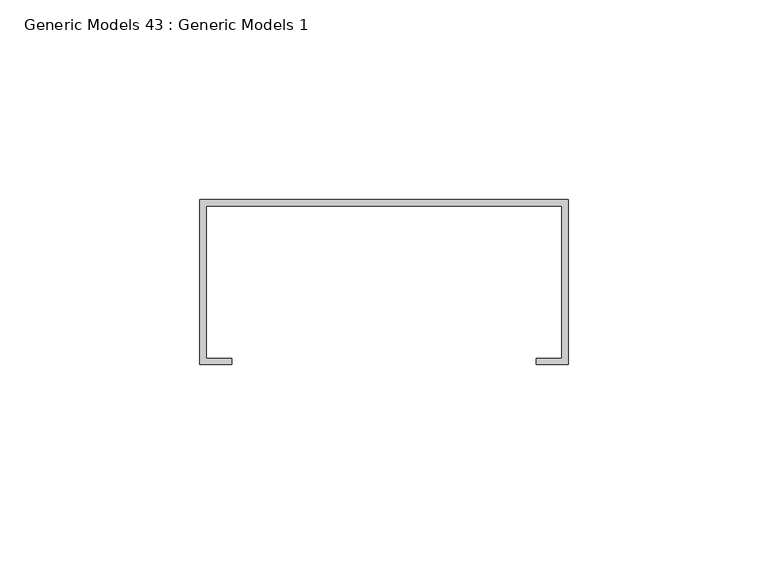
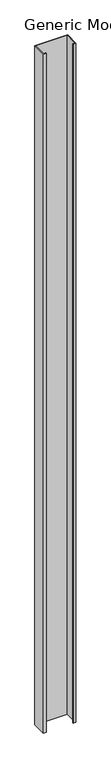
"""IFC4 building model written with IfcOpenShell, lengths in millimetres: proxy geometry, Generic Models 43 : Generic Models 1."""

import ifcopenshell
import ifcopenshell.guid

model = None  # the IFC model being written
_history = None  # IfcOwnerHistory: only IFC2X3 demands one
_inside = {}  # id of a spatial element -> (the spatial element, [elements in it])
_under = {}  # id of a project, library or spatial element -> (it, [spatial elements below it])
_declared = {}  # id of a project -> (the project, [libraries it declares])
_typed = {}  # id of a type object -> (the type object, [elements of that type])
_made_of = {}  # id of a material, layer set ... -> (it, [elements and type objects made of it])


def new_model(schema):
    """Start an empty IFC model of exactly this schema.

    Asked for "IFC4X3", IfcOpenShell would pick the latest addendum, in which some entities
    have other attributes; the version numbers below select the first issue.
    IFC2X3 requires an IfcOwnerHistory on every rooted entity: one is made here for all.
    """
    global model, _history
    if schema == "IFC4X3":
        model = ifcopenshell.file(schema_version=(4, 3, 0, 0))
    else:
        model = ifcopenshell.file(schema=schema)
    _inside.clear()
    _under.clear()
    _declared.clear()
    _typed.clear()
    _made_of.clear()
    _history = None
    if model.schema == "IFC2X3":
        org = make("IfcOrganization", Name="unknown")
        user = make(
            "IfcPersonAndOrganization",
            ThePerson=make("IfcPerson", FamilyName="unknown"),
            TheOrganization=org,
        )
        app = make(
            "IfcApplication",
            ApplicationDeveloper=org,
            Version="unknown",
            ApplicationFullName="unknown",
            ApplicationIdentifier="unknown",
        )
        _history = make(
            "IfcOwnerHistory",
            OwningUser=user,
            OwningApplication=app,
            ChangeAction="ADDED",
            CreationDate=0,
        )
    return model


def make(cls, **values):
    """One entity of the class cls with the attributes given. An attribute that is None is left unset."""
    return model.create_entity(
        cls, **{name: value for name, value in values.items() if value is not None}
    )


def rooted(cls, **values):
    """An entity with a GlobalId (a new one), such as an element, a storey or a relation."""
    return make(cls, GlobalId=ifcopenshell.guid.new(), OwnerHistory=_history, **values)


def si_unit(unit_type, name, prefix=None):
    """IfcSIUnit, for example si_unit("LENGTHUNIT", "METRE", prefix="MILLI")."""
    return make("IfcSIUnit", UnitType=unit_type, Prefix=prefix, Name=name)


def assignment(units):
    """IfcUnitAssignment: the units of a project."""
    return None if units is None else make("IfcUnitAssignment", Units=units)


def point(xyz):
    """IfcCartesianPoint."""
    return None if xyz is None else make("IfcCartesianPoint", Coordinates=xyz)


def direction(xyz):
    """IfcDirection."""
    return None if xyz is None else make("IfcDirection", DirectionRatios=xyz)


def frame(location, z_axis=None, x_axis=None):
    """IfcAxis2Placement3D, a coordinate frame: its origin and axes. An axis left out is left unset."""
    return make(
        "IfcAxis2Placement3D",
        Location=point(location),
        Axis=direction(z_axis),
        RefDirection=direction(x_axis),
    )


def origin():
    """The frame at (0, 0, 0) with its axes left unset."""
    return frame((0.0, 0.0, 0.0))


def place(relative_to, where):
    """IfcLocalPlacement: puts the frame where relative to a parent placement (None: the world)."""
    return make(
        "IfcLocalPlacement", PlacementRelTo=relative_to, RelativePlacement=where
    )


def context(
    kind, dimensions, precision=None, world=None, true_north=None, identifier=None
):
    """IfcGeometricRepresentationContext, for example the 3D "Model" context."""
    return make(
        "IfcGeometricRepresentationContext",
        ContextIdentifier=identifier,
        ContextType=kind,
        CoordinateSpaceDimension=dimensions,
        Precision=precision,
        WorldCoordinateSystem=world,
        TrueNorth=true_north,
    )


def project(units=None, contexts=None):
    """IfcProject with its units and contexts."""
    return rooted(
        "IfcProject",
        Name="project",
        RepresentationContexts=contexts,
        UnitsInContext=assignment(units),
    )


def spatial(cls, under=None, at=None, **own):
    """A site, building, storey or space (cls), placed at a placement, below another one or the project."""
    s = rooted(cls, ObjectPlacement=at, **own)
    if under is not None:
        _under.setdefault(under.id(), (under, []))[1].append(s)
    return s


def polyline(points):
    """IfcPolyline through the points."""
    return make("IfcPolyline", Points=[point(p) for p in points])


def outline(outer, holes=None, kind="AREA"):
    """IfcArbitraryClosedProfileDef: a profile drawn as a closed curve; with holes, ...WithVoids."""
    if holes is None:
        return make("IfcArbitraryClosedProfileDef", ProfileType=kind, OuterCurve=outer)
    return make(
        "IfcArbitraryProfileDefWithVoids",
        ProfileType=kind,
        OuterCurve=outer,
        InnerCurves=holes,
    )


def extrude(swept, where, along, depth):
    """IfcExtrudedAreaSolid: the profile swept, set in the frame where, extruded along a direction by depth."""
    return make(
        "IfcExtrudedAreaSolid",
        SweptArea=swept,
        Position=where,
        ExtrudedDirection=direction(along),
        Depth=depth,
    )


def shape(context_of_items, identifier, shape_type, items):
    """IfcShapeRepresentation: the items that make up one representation, for example the "Body"."""
    return make(
        "IfcShapeRepresentation",
        ContextOfItems=context_of_items,
        RepresentationIdentifier=identifier,
        RepresentationType=shape_type,
        Items=items,
    )


def source(mapping_origin, context_of_items, identifier, shape_type, items):
    """IfcRepresentationMap: a shape defined once, which mapped items show again and again."""
    return make(
        "IfcRepresentationMap",
        MappingOrigin=mapping_origin,
        MappedRepresentation=shape(context_of_items, identifier, shape_type, items),
    )


def transform(
    local_origin,
    x_axis=None,
    y_axis=None,
    z_axis=None,
    scale=None,
    scale2=None,
    scale3=None,
    uniform=True,
):
    """IfcCartesianTransformationOperator3D, or its non-uniform kind. x_axis, y_axis, z_axis: its Axis1, 2, 3."""
    if uniform:
        return make(
            "IfcCartesianTransformationOperator3D",
            Axis1=direction(x_axis),
            Axis2=direction(y_axis),
            LocalOrigin=point(local_origin),
            Scale=scale,
            Axis3=direction(z_axis),
        )
    return make(
        "IfcCartesianTransformationOperator3DnonUniform",
        Axis1=direction(x_axis),
        Axis2=direction(y_axis),
        LocalOrigin=point(local_origin),
        Scale=scale,
        Axis3=direction(z_axis),
        Scale2=scale2,
        Scale3=scale3,
    )


def mapped(mapping_source, mapping_target):
    """IfcMappedItem: shows the shape of a source again, moved by a transform."""
    return make(
        "IfcMappedItem", MappingSource=mapping_source, MappingTarget=mapping_target
    )


def made_of(thing, what):
    """Note that an element or type object is made of a material, layer set ...; save() writes the relation."""
    if what is not None:
        _made_of.setdefault(what.id(), (what, []))[1].append(thing)
    return thing


def element(
    cls,
    number,
    at=None,
    inside=None,
    cuts=None,
    type_object=None,
    material=None,
    context=None,
    identifier="Body",
    shape_type=None,
    held_by="IfcProductDefinitionShape",
    body=None,
    shapes=None,
    **own,
):
    """One element of the class cls, such as IfcWall. Its Tag is "e" and its number.

    at: its placement. inside: the storey or other place that contains it. cuts: it is an
    opening in that element (IfcRelVoidsElement). A single representation is given by context,
    identifier, shape_type and body (its items); several are given by shapes. held_by: the class
    of the entity that holds the representations. save() writes the other relations.
    """
    e = rooted(cls, Tag="e%d" % number, ObjectPlacement=at, **own)
    if body is not None:
        shapes = [shape(context, identifier, shape_type, body)]
    if shapes is not None:
        e.Representation = make(held_by, Representations=shapes)
    if inside is not None:
        _inside.setdefault(inside.id(), (inside, []))[1].append(e)
    if cuts is not None:
        rooted(
            "IfcRelVoidsElement", RelatingBuildingElement=cuts, RelatedOpeningElement=e
        )
    if type_object is not None:
        _typed.setdefault(type_object.id(), (type_object, []))[1].append(e)
    return made_of(e, material)


def aggregate(whole, parts):
    """IfcRelAggregates: a whole, such as a stair, and the parts it consists of."""
    return rooted("IfcRelAggregates", RelatingObject=whole, RelatedObjects=parts)


def save(model, path):
    """Write the relations noted so far, then the file.

    IfcRelAggregates (storeys below a building ...), IfcRelContainedInSpatialStructure (elements
    in a storey), IfcRelDefinesByType, IfcRelAssociatesMaterial and IfcRelDeclares: one each for
    every whole, place, type object, material and project.
    """
    for whole, parts in _under.values():
        aggregate(whole, parts)
    for where, things in _inside.values():
        rooted(
            "IfcRelContainedInSpatialStructure",
            RelatedElements=things,
            RelatingStructure=where,
        )
    for kind, things in _typed.values():
        rooted("IfcRelDefinesByType", RelatedObjects=things, RelatingType=kind)
    for what, things in _made_of.values():
        rooted("IfcRelAssociatesMaterial", RelatedObjects=things, RelatingMaterial=what)
    for by, libraries in _declared.values():
        rooted("IfcRelDeclares", RelatingContext=by, RelatedDefinitions=libraries)
    model.write(path)


def generic_models_43_generic_models_1_113e5eee(model_context):
    return source(origin(), model_context, "Body", "SweptSolid", [
        extrude(outline(polyline([(51003.2, 630.2375), (51003.2, 588.9625), (50995.2625, 588.9625), (50995.2625, 590.55), (51001.6125, 590.55), (51001.6125, 628.65), (50912.7125, 628.65), (50912.7125, 590.55), (50919.0625, 590.55), (50919.0625, 588.9625), (50911.125, 588.9625), (50911.125, 630.2375), (51003.2, 630.2375)])), frame((0.0, 0.0, 1.5875), z_axis=(0.0, 0.0, 1.0), x_axis=(1.0, 0.0, 0.0)), (0.0, 0.0, 1.0), 2025.65),
    ])


if __name__ == "__main__":
    model = new_model("IFC4")
    model_context = context("Model", 3, world=origin())
    ifc_project = project(units=[si_unit("LENGTHUNIT", "METRE", prefix="MILLI")], contexts=[model_context])
    site = spatial("IfcSite", under=ifc_project)
    building = spatial("IfcBuilding", under=site)
    placement = place(None, origin())
    generic_models_43_generic_models_1_shape = generic_models_43_generic_models_1_113e5eee(model_context)
    element("IfcBuildingElementProxy", 1, Name="Generic Models 43 : Generic Models 1", ObjectType="Generic Models 43 : Generic Models 1", at=placement, inside=building, context=model_context, shape_type="MappedRepresentation", body=[
        mapped(generic_models_43_generic_models_1_shape, transform((0.0, 0.0, 0.0), x_axis=(1.0, 0.0, 0.0), y_axis=(0.0, 1.0, 0.0), z_axis=(0.0, 0.0, 1.0))),
    ])
    save(model, "model.ifc")

# Revit data of these elements
# Element 1 (IfcBuildingElementProxy, "Generic Models 43 : Generic Models 1")
#   Materials on its faces: "METAL STUDS (MATCH EXISTING SIZE/GAUGE/SPACING)"
# Materials
#   "METAL STUDS (MATCH EXISTING SIZE/GAUGE/SPACING)": class "Unassigned", colour RGB 210 209 208, transparency 0, Keynote = "M05121300.02", Cost = 0
